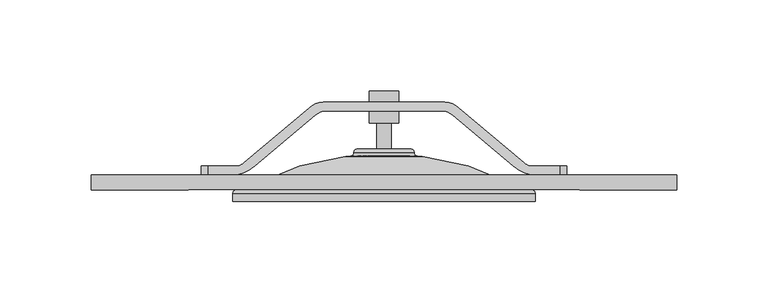
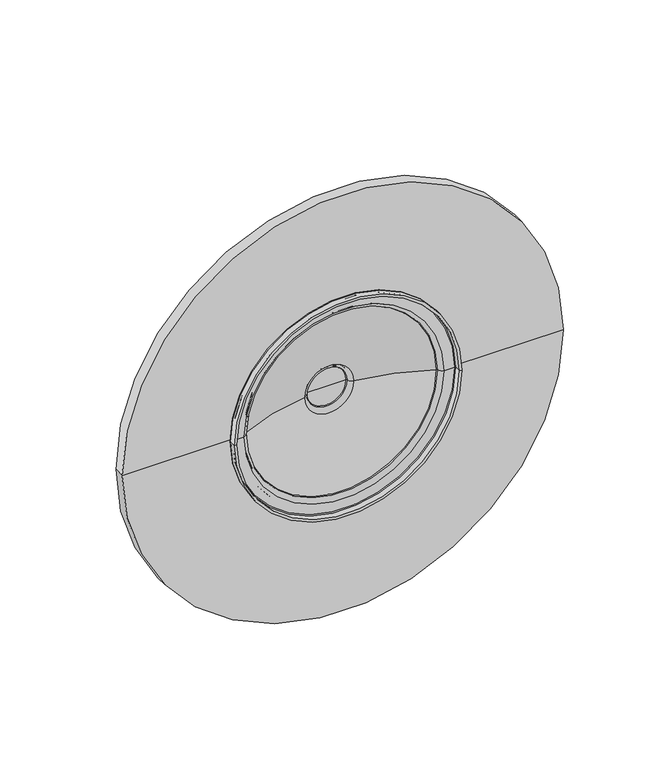
"""IFC4 building model written with IfcOpenShell, lengths in millimetres: proxy geometry, BVNC 300 8Y. : BVNC 300 8Y."""

from ifc_helpers import new_model, si_unit, point, frame, origin, place, context, project, spatial, polyline, circle_curve, ellipse_curve, trimmed, source, transform, mapped, element, save
from ifc_brep_helpers import plane_surface, cylinder_surface, revolved_surface, advanced_brep


def mechanical_equipment_492a67d3(model_context):
    return source(origin(), model_context, "Body", "AdvancedBrep", [
        advanced_brep(
        [(44.3795006, 108.0, 2610.0), (54.2298211, 113.0, 2610.0), (87.44309, 140.8692417, 2610.0), (91.8102497, 143.0, 2610.0), (125.0, 143.0, 2610.0), (158.1897503, 143.0, 2610.0), (162.55691, 140.8692417, 2610.0), (195.7701789, 113.0, 2610.0), (205.6204994, 108.0, 2610.0), (221.2200072, 108.0, 2610.0), (221.2200072, 113.0, 2610.0), (205.6204994, 113.0, 2610.0), (201.5540671, 114.8851429, 2610.0), (165.874925, 144.8234979, 2610.0), (158.1897503, 148.0, 2610.0), (125.0, 148.0, 2610.0), (91.8102497, 148.0, 2610.0), (84.125075, 144.8234979, 2610.0), (48.4459329, 114.8851429, 2610.0), (44.3795006, 113.0, 2610.0), (28.7799928, 113.0, 2610.0), (28.7799928, 108.0, 2610.0), (44.3795006, 113.0, 2590.0), (48.4459329, 114.8851429, 2590.0), (84.125075, 144.8234979, 2590.0), (91.8102497, 148.0, 2590.0), (125.0, 148.0, 2590.0), (158.1897503, 148.0, 2590.0), (165.874925, 144.8234979, 2590.0), (201.5540671, 114.8851429, 2590.0), (205.6204994, 113.0, 2590.0), (221.2200072, 113.0, 2590.0), (221.2200072, 108.0, 2590.0), (205.6204994, 108.0, 2590.0), (195.7701789, 113.0, 2590.0), (162.55691, 140.8692417, 2590.0), (158.1897503, 143.0, 2590.0), (125.0, 143.0, 2590.0), (91.8102497, 143.0, 2590.0), (87.44309, 140.8692417, 2590.0), (54.2298211, 113.0, 2590.0), (44.3795006, 108.0, 2590.0), (28.7799928, 108.0, 2590.0), (28.7799928, 113.0, 2590.0), (25.0, 108.0, 2606.2200072), (25.0, 108.0, 2593.7799928), (225.0, 108.0, 2593.7799928), (225.0, 108.0, 2606.2200072), (225.0, 113.0, 2593.7799928), (225.0, 113.0, 2606.2200072), (25.0, 113.0, 2593.7799928), (25.0, 113.0, 2606.2200072)],
        [
            (0, 1, circle_curve(frame((38.5511411, 131.6851233, 2610.0), z_axis=(0.0, 0.0, 1.0), x_axis=(1.0, 0.0, 0.0)), 24.3916961)),
            (1, 2),
            (2, 3, circle_curve(frame((93.9022065, 133.1715663, 2610.0), z_axis=(0.0, 0.0, -1.0), x_axis=(1.0, 0.0, 0.0)), 10.0486015)),
            (3, 4),
            (4, 5),
            (5, 6, circle_curve(frame((156.0977935, 133.1715663, 2610.0), z_axis=(0.0, 0.0, -1.0), x_axis=(-1.0, 0.0, 0.0)), 10.0486015)),
            (6, 7),
            (7, 8, circle_curve(frame((211.4488589, 131.6851233, 2610.0), z_axis=(0.0, 0.0, 1.0), x_axis=(-1.0, 0.0, 0.0)), 24.3916961)),
            (8, 9),
            (9, 10),
            (10, 11),
            (11, 12, circle_curve(frame((205.6204994, 118.3284116, 2610.0), z_axis=(0.0, 0.0, -1.0), x_axis=(-1.0, 0.0, 0.0)), 5.3284116)),
            (12, 13),
            (13, 14, circle_curve(frame((158.1897503, 137.115059, 2610.0), z_axis=(0.0, 0.0, 1.0), x_axis=(-1.0, 0.0, 0.0)), 10.884941)),
            (14, 15),
            (15, 16),
            (16, 17, circle_curve(frame((91.8102497, 137.115059, 2610.0), z_axis=(0.0, 0.0, 1.0), x_axis=(1.0, 0.0, 0.0)), 10.884941)),
            (17, 18),
            (18, 19, circle_curve(frame((44.3795006, 118.3284116, 2610.0), z_axis=(0.0, 0.0, -1.0), x_axis=(1.0, 0.0, 0.0)), 5.3284116)),
            (19, 20),
            (20, 21),
            (21, 0),
            (22, 23, circle_curve(frame((44.3795006, 118.3284116, 2590.0), z_axis=(0.0, 0.0, 1.0), x_axis=(1.0, 0.0, 0.0)), 5.3284116)),
            (23, 24),
            (24, 25, circle_curve(frame((91.8102497, 137.115059, 2590.0), z_axis=(0.0, 0.0, -1.0), x_axis=(1.0, 0.0, 0.0)), 10.884941)),
            (25, 26),
            (26, 27),
            (27, 28, circle_curve(frame((158.1897503, 137.115059, 2590.0), z_axis=(0.0, 0.0, -1.0), x_axis=(-1.0, 0.0, 0.0)), 10.884941)),
            (28, 29),
            (29, 30, circle_curve(frame((205.6204994, 118.3284116, 2590.0), z_axis=(0.0, 0.0, 1.0), x_axis=(-1.0, 0.0, 0.0)), 5.3284116)),
            (30, 31),
            (31, 32),
            (32, 33),
            (33, 34, circle_curve(frame((211.4488589, 131.6851233, 2590.0), z_axis=(0.0, 0.0, -1.0), x_axis=(-1.0, 0.0, 0.0)), 24.3916961)),
            (34, 35),
            (35, 36, circle_curve(frame((156.0977935, 133.1715663, 2590.0), z_axis=(0.0, 0.0, 1.0), x_axis=(-1.0, 0.0, 0.0)), 10.0486015)),
            (36, 37),
            (37, 38),
            (38, 39, circle_curve(frame((93.9022065, 133.1715663, 2590.0), z_axis=(0.0, 0.0, 1.0), x_axis=(1.0, 0.0, 0.0)), 10.0486015)),
            (39, 40),
            (40, 41, circle_curve(frame((38.5511411, 131.6851233, 2590.0), z_axis=(0.0, 0.0, -1.0), x_axis=(1.0, 0.0, 0.0)), 24.3916961)),
            (41, 42),
            (42, 43),
            (43, 22),
            (41, 0),
            (21, 44, circle_curve(frame((28.7799928, 108.0, 2606.2200072), z_axis=(0.0, -1.0, 0.0), x_axis=(1.0, 0.0, 0.0)), 3.7799928)),
            (44, 45),
            (45, 42, circle_curve(frame((28.7799928, 108.0, 2593.7799928), z_axis=(0.0, -1.0, 0.0), x_axis=(1.0, 0.0, 0.0)), 3.7799928)),
            (40, 1),
            (39, 2),
            (38, 3),
            (37, 4),
            (36, 5),
            (35, 6),
            (34, 7),
            (33, 8),
            (32, 46, circle_curve(frame((221.2200072, 108.0, 2593.7799928), z_axis=(0.0, -1.0, 0.0), x_axis=(-1.0, 0.0, 0.0)), 3.7799928)),
            (46, 47),
            (47, 9, circle_curve(frame((221.2200072, 108.0, 2606.2200072), z_axis=(0.0, -1.0, 0.0), x_axis=(-1.0, 0.0, 0.0)), 3.7799928)),
            (46, 48),
            (48, 49),
            (49, 47),
            (30, 11),
            (10, 49, circle_curve(frame((221.2200072, 113.0, 2606.2200072), z_axis=(0.0, 1.0, 0.0), x_axis=(-1.0, 0.0, 0.0)), 3.7799928)),
            (48, 31, circle_curve(frame((221.2200072, 113.0, 2593.7799928), z_axis=(0.0, 1.0, 0.0), x_axis=(-1.0, 0.0, 0.0)), 3.7799928)),
            (29, 12),
            (28, 13),
            (27, 14),
            (26, 15),
            (25, 16),
            (24, 17),
            (23, 18),
            (22, 19),
            (43, 50, circle_curve(frame((28.7799928, 113.0, 2593.7799928), z_axis=(0.0, 1.0, 0.0), x_axis=(1.0, 0.0, 0.0)), 3.7799928)),
            (50, 51),
            (51, 20, circle_curve(frame((28.7799928, 113.0, 2606.2200072), z_axis=(0.0, 1.0, 0.0), x_axis=(1.0, 0.0, 0.0)), 3.7799928)),
            (44, 51),
            (50, 45),
        ],
        [
            plane_surface(frame((25.0, 108.0, 2610.0), z_axis=(0.0, 0.0, 1.0), x_axis=(1.0, 0.0, 0.0))),
            plane_surface(frame((25.0, 108.0, 2590.0), z_axis=(0.0, 0.0, -1.0), x_axis=(-1.0, 0.0, 0.0))),
            plane_surface(frame((25.0, 108.0, 2610.0), z_axis=(0.0, -1.0, 0.0), x_axis=(0.0, 0.0, -1.0))),
            cylinder_surface(frame((38.5511411, 131.6851233, 2590.0), z_axis=(0.0, 0.0, 1.0), x_axis=(1.0, 0.0, 0.0)), 24.3916961),
            plane_surface(frame((54.2298211, 113.0, 2610.0), z_axis=(0.6427876096865391, -0.7660444431189783, 0.0), x_axis=(0.0, 0.0, -1.0))),
            revolved_surface(polyline([(103.95080800000001, 133.1715663, 2590.0), (103.95080800000001, 133.1715663, 2610.0)]), (93.9022065, 133.1715663, 2590.0), (0.0, 0.0, -1.0)),
            plane_surface(frame((91.8102497, 143.0, 2610.0), z_axis=(0.0, -1.0, 0.0), x_axis=(0.0, 0.0, -1.0))),
            plane_surface(frame((125.0, 143.0, 2610.0), z_axis=(0.0, -1.0, 0.0), x_axis=(0.0, 0.0, -1.0))),
            revolved_surface(polyline([(146.049192, 133.1715663, 2590.0), (146.049192, 133.1715663, 2610.0)]), (156.0977935, 133.1715663, 2590.0), (0.0, 0.0, -1.0)),
            plane_surface(frame((162.55691, 140.8692417, 2610.0), z_axis=(-0.6427876096865387, -0.7660444431189786, 0.0), x_axis=(0.0, 0.0, -1.0))),
            cylinder_surface(frame((211.4488589, 131.6851233, 2590.0), z_axis=(0.0, 0.0, 1.0), x_axis=(-1.0, 0.0, 0.0)), 24.3916961),
            plane_surface(frame((205.6204994, 108.0, 2610.0), z_axis=(0.0, -1.0, 0.0), x_axis=(0.0, 0.0, -1.0))),
            plane_surface(frame((225.0, 108.0, 2610.0), z_axis=(1.0, 0.0, 0.0), x_axis=(0.0, 0.0, -1.0))),
            plane_surface(frame((225.0, 113.0, 2610.0), z_axis=(0.0, 1.0, 0.0), x_axis=(0.0, 0.0, -1.0))),
            revolved_surface(polyline([(200.2920878, 118.3284116, 2590.0), (200.2920878, 118.3284116, 2610.0)]), (205.6204994, 118.3284116, 2590.0), (0.0, 0.0, -1.0)),
            plane_surface(frame((201.5540671, 114.8851429, 2610.0), z_axis=(0.6427876096865414, 0.7660444431189763, 0.0), x_axis=(0.0, 0.0, -1.0))),
            cylinder_surface(frame((158.1897503, 137.115059, 2590.0), z_axis=(0.0, 0.0, 1.0), x_axis=(-1.0, 0.0, 0.0)), 10.884941),
            plane_surface(frame((158.1897503, 148.0, 2610.0), z_axis=(0.0, 1.0, 0.0), x_axis=(0.0, 0.0, -1.0))),
            plane_surface(frame((125.0, 148.0, 2610.0), z_axis=(0.0, 1.0, 0.0), x_axis=(0.0, 0.0, -1.0))),
            cylinder_surface(frame((91.8102497, 137.115059, 2590.0), z_axis=(0.0, 0.0, 1.0), x_axis=(1.0, 0.0, 0.0)), 10.884941),
            plane_surface(frame((84.125075, 144.8234979, 2610.0), z_axis=(-0.6427876096865359, 0.766044443118981, 0.0), x_axis=(0.0, 0.0, -1.0))),
            revolved_surface(polyline([(49.7079122, 118.3284116, 2590.0), (49.7079122, 118.3284116, 2610.0)]), (44.3795006, 118.3284116, 2590.0), (0.0, 0.0, -1.0)),
            plane_surface(frame((44.3795006, 113.0, 2610.0), z_axis=(0.0, 1.0, 0.0), x_axis=(0.0, 0.0, -1.0))),
            plane_surface(frame((25.0, 113.0, 2610.0), z_axis=(-1.0, 0.0, 0.0), x_axis=(0.0, 0.0, -1.0))),
            cylinder_surface(frame((28.7799928, 108.0, 2593.7799928), z_axis=(0.0, -1.0, 0.0), x_axis=(1.0, 0.0, 0.0)), 3.7799928),
            cylinder_surface(frame((28.7799928, 93.5, 2606.2200072), z_axis=(0.0, -1.0, 0.0), x_axis=(1.0, 0.0, 0.0)), 3.7799928),
            cylinder_surface(frame((221.2200072, 93.5, 2593.7799928), z_axis=(0.0, -1.0, 0.0), x_axis=(-1.0, 0.0, 0.0)), 3.7799928),
            cylinder_surface(frame((221.2200072, 93.5, 2606.2200072), z_axis=(0.0, -1.0, 0.0), x_axis=(-1.0, 0.0, 0.0)), 3.7799928),
        ],
        [
            (0, [[1, 2, 3, 4, 5, 6, 7, 8, 9, 10, 11, 12, 13, 14, 15, 16, 17, 18, 19, 20, 21, 22]]),
            (1, [[23, 24, 25, 26, 27, 28, 29, 30, 31, 32, 33, 34, 35, 36, 37, 38, 39, 40, 41, 42, 43, 44]]),
            (2, [[45, -22, 46, 47, 48, -42]]),
            (3, [[-1, -45, -41, 49]]),
            (4, [[-2, -49, -40, 50]]),
            (5, [[-3, -50, -39, 51]]),
            (6, [[-4, -51, -38, 52]]),
            (7, [[-5, -52, -37, 53]]),
            (8, [[-6, -53, -36, 54]]),
            (9, [[-7, -54, -35, 55]]),
            (10, [[-8, -55, -34, 56]]),
            (11, [[-56, -33, 57, 58, 59, -9]]),
            (12, [[-58, 60, 61, 62]]),
            (13, [[63, -11, 64, -61, 65, -31]]),
            (14, [[-12, -63, -30, 66]]),
            (15, [[-13, -66, -29, 67]]),
            (16, [[-14, -67, -28, 68]]),
            (17, [[-15, -68, -27, 69]]),
            (18, [[-16, -69, -26, 70]]),
            (19, [[-17, -70, -25, 71]]),
            (20, [[-18, -71, -24, 72]]),
            (21, [[-19, -72, -23, 73]]),
            (22, [[-73, -44, 74, 75, 76, -20]]),
            (23, [[-47, 77, -75, 78]]),
            (24, [[-43, -48, -78, -74]]),
            (25, [[-21, -76, -77, -46]]),
            (26, [[-32, -65, -60, -57]]),
            (27, [[-10, -59, -62, -64]]),
        ],
    ),
        advanced_brep(
        [(207.7271571, 93.5, 2600.0), (42.2728429, 93.5, 2600.0), (42.2728429, 97.7728429, 2600.0), (207.7271571, 97.7728429, 2600.0), (205.9367462, 93.5, 2600.0), (44.0632538, 93.5, 2600.0), (205.9367462, 97.9071057, 2600.0), (44.0632538, 97.9071057, 2600.0), (205.3438519, 98.5, 2600.0), (44.6561481, 98.5, 2600.0), (197.7785514, 98.5, 2600.0), (52.2214486, 98.5, 2600.0), (194.5390342, 101.1233093, 2600.0), (55.4609658, 101.1233093, 2600.0), (194.110594, 101.9290881, 2600.0), (55.889406, 101.9290881, 2600.0), (143.1174907, 117.056758, 2600.0), (106.8825093, 117.056758, 2600.0), (139.9690463, 120.2052024, 2600.0), (110.0309537, 120.2052024, 2600.0), (139.3942487, 120.78, 2600.0), (110.6057513, 120.78, 2600.0), (125.0, 120.78, 2600.0), (139.6388233, 122.2731901, 2600.0), (110.3611767, 122.2731901, 2600.0), (120.9566338, 122.2731901, 2600.0), (129.0433662, 122.2731901, 2600.0), (141.5029828, 120.4090307, 2600.0), (108.4970172, 120.4090307, 2600.0), (143.1991524, 118.522856, 2600.0), (106.8008476, 118.522856, 2600.0), (145.9642188, 118.2410596, 2600.0), (104.0357812, 118.2410596, 2600.0), (194.877574, 103.206216, 2600.0), (55.122426, 103.206216, 2600.0), (196.1038029, 101.6367146, 2600.0), (53.8961971, 101.6367146, 2600.0), (198.0543634, 100.0, 2600.0), (51.9456366, 100.0, 2600.0), (200.0, 100.0, 2600.0), (50.0, 100.0, 2600.0), (200.0, 108.0, 2600.0), (50.0, 108.0, 2600.0), (285.0, 108.0, 2600.0), (-35.0, 108.0, 2600.0), (285.0, 100.0, 2600.0), (-35.0, 100.0, 2600.0), (205.5, 100.0, 2600.0), (44.5, 100.0, 2600.0), (133.0867323, 136.6576943, 2600.0), (116.9132677, 136.6576943, 2600.0), (116.9132677, 153.9, 2600.0), (133.0867323, 153.9, 2600.0), (129.0433662, 136.6576943, 2600.0), (120.9566338, 136.6576943, 2600.0), (125.0, 153.9, 2600.0)],
        [
            (0, 1, circle_curve(frame((125.0, 93.5, 2600.0), z_axis=(0.0, 1.0, 0.0), x_axis=(-1.0, 0.0, 0.0)), 82.7271571)),
            (1, 2),
            (2, 3, circle_curve(frame((125.0, 97.7728429, 2600.0), z_axis=(0.0, -1.0, 0.0), x_axis=(-1.0, 0.0, 0.0)), 82.7271571)),
            (3, 0),
            (1, 0, circle_curve(frame((125.0, 93.5, 2600.0), z_axis=(0.0, 1.0, 0.0), x_axis=(-1.0, 0.0, 0.0)), 82.7271571)),
            (3, 2, circle_curve(frame((125.0, 97.7728429, 2600.0), z_axis=(0.0, -1.0, 0.0), x_axis=(-1.0, 0.0, 0.0)), 82.7271571)),
            (0, 4),
            (4, 5, circle_curve(frame((125.0, 93.5, 2600.0), z_axis=(0.0, 1.0, 0.0), x_axis=(-1.0, 0.0, 0.0)), 80.9367462)),
            (5, 1),
            (5, 4, circle_curve(frame((125.0, 93.5, 2600.0), z_axis=(0.0, 1.0, 0.0), x_axis=(-1.0, 0.0, 0.0)), 80.9367462)),
            (4, 6),
            (6, 7, circle_curve(frame((125.0, 97.9071057, 2600.0), z_axis=(0.0, 1.0, 0.0), x_axis=(-1.0, 0.0, 0.0)), 80.9367462)),
            (7, 5),
            (7, 6, circle_curve(frame((125.0, 97.9071057, 2600.0), z_axis=(0.0, 1.0, 0.0), x_axis=(-1.0, 0.0, 0.0)), 80.9367462)),
            (6, 8, circle_curve(frame((205.3438519, 97.9071057, 2600.0), z_axis=(0.0, 0.0, 1.0), x_axis=(-1.0, 0.0, 0.0)), 0.5928943)),
            (8, 9, circle_curve(frame((125.0, 98.5, 2600.0), z_axis=(0.0, 1.0, 0.0), x_axis=(-1.0, 0.0, 0.0)), 80.3438519)),
            (9, 7, circle_curve(frame((44.6561481, 97.9071057, 2600.0), z_axis=(0.0, 0.0, 1.0), x_axis=(1.0, 0.0, 0.0)), 0.5928943)),
            (9, 8, circle_curve(frame((125.0, 98.5, 2600.0), z_axis=(0.0, 1.0, 0.0), x_axis=(-1.0, 0.0, 0.0)), 80.3438519)),
            (8, 10),
            (10, 11, circle_curve(frame((125.0, 98.5, 2600.0), z_axis=(0.0, 1.0, 0.0), x_axis=(-1.0, 0.0, 0.0)), 72.7785514)),
            (11, 9),
            (11, 10, circle_curve(frame((125.0, 98.5, 2600.0), z_axis=(0.0, 1.0, 0.0), x_axis=(-1.0, 0.0, 0.0)), 72.7785514)),
            (10, 12, circle_curve(frame((197.9467336, 102.0195777, 2600.0), z_axis=(0.0, 0.0, -1.0), x_axis=(-1.0, 0.0, 0.0)), 3.5235937)),
            (12, 13, circle_curve(frame((125.0, 101.1233093, 2600.0), z_axis=(0.0, 1.0, 0.0), x_axis=(-1.0, 0.0, 0.0)), 69.5390342)),
            (13, 11, circle_curve(frame((52.0532664, 102.0195777, 2600.0), z_axis=(0.0, 0.0, -1.0), x_axis=(1.0, 0.0, 0.0)), 3.5235937)),
            (13, 12, circle_curve(frame((125.0, 101.1233093, 2600.0), z_axis=(0.0, 1.0, 0.0), x_axis=(-1.0, 0.0, 0.0)), 69.5390342)),
            (12, 14, circle_curve(frame((193.7458269, 101.2183458, 2600.0), z_axis=(0.0, 0.0, 1.0), x_axis=(-1.0, 0.0, 0.0)), 0.7988803)),
            (14, 15, circle_curve(frame((125.0, 101.9290881, 2600.0), z_axis=(0.0, 1.0, 0.0), x_axis=(-1.0, 0.0, 0.0)), 69.110594)),
            (15, 13, circle_curve(frame((56.2541731, 101.2183458, 2600.0), z_axis=(0.0, 0.0, 1.0), x_axis=(1.0, 0.0, 0.0)), 0.7988803)),
            (15, 14, circle_curve(frame((125.0, 101.9290881, 2600.0), z_axis=(0.0, 1.0, 0.0), x_axis=(-1.0, 0.0, 0.0)), 69.110594)),
            (14, 16, circle_curve(frame((128.3688639, -26.1675298, 2600.0), z_axis=(0.0, 0.0, 1.0), x_axis=(-1.0, 0.0, 0.0)), 143.9816606)),
            (16, 17, circle_curve(frame((125.0, 117.056758, 2600.0), z_axis=(0.0, 1.0, 0.0), x_axis=(-1.0, 0.0, 0.0)), 18.1174907)),
            (17, 15, circle_curve(frame((121.6311361, -26.1675298, 2600.0), z_axis=(0.0, 0.0, 1.0), x_axis=(1.0, 0.0, 0.0)), 143.9816606)),
            (17, 16, circle_curve(frame((125.0, 117.056758, 2600.0), z_axis=(0.0, 1.0, 0.0), x_axis=(-1.0, 0.0, 0.0)), 18.1174907)),
            (16, 18, circle_curve(frame((143.1174907, 120.2052024, 2600.0), z_axis=(0.0, 0.0, -1.0), x_axis=(-1.0, 0.0, 0.0)), 3.1484444)),
            (18, 19, circle_curve(frame((125.0, 120.2052024, 2600.0), z_axis=(0.0, 1.0, 0.0), x_axis=(-1.0, 0.0, 0.0)), 14.9690463)),
            (19, 17, circle_curve(frame((106.8825093, 120.2052024, 2600.0), z_axis=(0.0, 0.0, -1.0), x_axis=(1.0, 0.0, 0.0)), 3.1484444)),
            (19, 18, circle_curve(frame((125.0, 120.2052024, 2600.0), z_axis=(0.0, 1.0, 0.0), x_axis=(-1.0, 0.0, 0.0)), 14.9690463)),
            (18, 20, circle_curve(frame((139.3942487, 120.2052024, 2600.0), z_axis=(0.0, 0.0, 1.0), x_axis=(-1.0, 0.0, 0.0)), 0.5747976)),
            (20, 21, circle_curve(frame((125.0, 120.78, 2600.0), z_axis=(0.0, 1.0, 0.0), x_axis=(-1.0, 0.0, 0.0)), 14.3942487)),
            (21, 19, circle_curve(frame((110.6057513, 120.2052024, 2600.0), z_axis=(0.0, 0.0, 1.0), x_axis=(1.0, 0.0, 0.0)), 0.5747976)),
            (21, 20, circle_curve(frame((125.0, 120.78, 2600.0), z_axis=(0.0, 1.0, 0.0), x_axis=(-1.0, 0.0, 0.0)), 14.3942487)),
            (20, 22),
            (22, 21),
            (23, 24, circle_curve(frame((125.0, 122.2731901, 2600.0), z_axis=(0.0, 1.0, 0.0), x_axis=(-1.0, 0.0, 0.0)), 14.6388233)),
            (24, 25),
            (25, 26, circle_curve(frame((125.0, 122.2731901, 2600.0), z_axis=(0.0, -1.0, 0.0), x_axis=(-1.0, 0.0, 0.0)), 4.0433662)),
            (26, 23),
            (24, 23, circle_curve(frame((125.0, 122.2731901, 2600.0), z_axis=(0.0, 1.0, 0.0), x_axis=(-1.0, 0.0, 0.0)), 14.6388233)),
            (26, 25, circle_curve(frame((125.0, 122.2731901, 2600.0), z_axis=(0.0, -1.0, 0.0), x_axis=(-1.0, 0.0, 0.0)), 4.0433662)),
            (23, 27, circle_curve(frame((139.6388233, 120.4090307, 2600.0), z_axis=(0.0, 0.0, -1.0), x_axis=(-1.0, 0.0, 0.0)), 1.8641595)),
            (27, 28, circle_curve(frame((125.0, 120.4090307, 2600.0), z_axis=(0.0, 1.0, 0.0), x_axis=(-1.0, 0.0, 0.0)), 16.5029828)),
            (28, 24, circle_curve(frame((110.3611767, 120.4090307, 2600.0), z_axis=(0.0, 0.0, -1.0), x_axis=(1.0, 0.0, 0.0)), 1.8641595)),
            (28, 27, circle_curve(frame((125.0, 120.4090307, 2600.0), z_axis=(0.0, 1.0, 0.0), x_axis=(-1.0, 0.0, 0.0)), 16.5029828)),
            (27, 29, circle_curve(frame((143.3997997, 120.4090307, 2600.0), z_axis=(0.0, 0.0, 1.0), x_axis=(-1.0, 0.0, 0.0)), 1.8968169)),
            (29, 30, circle_curve(frame((125.0, 118.522856, 2600.0), z_axis=(0.0, 1.0, 0.0), x_axis=(-1.0, 0.0, 0.0)), 18.1991524)),
            (30, 28, circle_curve(frame((106.6002003, 120.4090307, 2600.0), z_axis=(0.0, 0.0, 1.0), x_axis=(1.0, 0.0, 0.0)), 1.8968169)),
            (30, 29, circle_curve(frame((125.0, 118.522856, 2600.0), z_axis=(0.0, 1.0, 0.0), x_axis=(-1.0, 0.0, 0.0)), 18.1991524)),
            (29, 31, circle_curve(frame((176.4809645, 431.386753, 2600.0), z_axis=(0.0, 0.0, 1.0), x_axis=(-1.0, 0.0, 0.0)), 314.6291421)),
            (31, 32, circle_curve(frame((125.0, 118.2410596, 2600.0), z_axis=(0.0, 1.0, 0.0), x_axis=(-1.0, 0.0, 0.0)), 20.9642188)),
            (32, 30, circle_curve(frame((73.5190355, 431.386753, 2600.0), z_axis=(0.0, 0.0, 1.0), x_axis=(1.0, 0.0, 0.0)), 314.6291421)),
            (32, 31, circle_curve(frame((125.0, 118.2410596, 2600.0), z_axis=(0.0, 1.0, 0.0), x_axis=(-1.0, 0.0, 0.0)), 20.9642188)),
            (31, 33, circle_curve(frame((131.9555378, -14.4169888, 2600.0), z_axis=(0.0, 0.0, -1.0), x_axis=(-1.0, 0.0, 0.0)), 133.3956557)),
            (33, 34, circle_curve(frame((125.0, 103.206216, 2600.0), z_axis=(0.0, 1.0, 0.0), x_axis=(-1.0, 0.0, 0.0)), 69.877574)),
            (34, 32, circle_curve(frame((118.0444622, -14.4169888, 2600.0), z_axis=(0.0, 0.0, -1.0), x_axis=(1.0, 0.0, 0.0)), 133.3956557)),
            (34, 33, circle_curve(frame((125.0, 103.206216, 2600.0), z_axis=(0.0, 1.0, 0.0), x_axis=(-1.0, 0.0, 0.0)), 69.877574)),
            (33, 35, circle_curve(frame((194.0147871, 101.2683648, 2600.0), z_axis=(0.0, 0.0, -1.0), x_axis=(-1.0, 0.0, 0.0)), 2.1212422)),
            (35, 36, circle_curve(frame((125.0, 101.6367146, 2600.0), z_axis=(0.0, 1.0, 0.0), x_axis=(-1.0, 0.0, 0.0)), 71.1038029)),
            (36, 34, circle_curve(frame((55.9852129, 101.2683648, 2600.0), z_axis=(0.0, 0.0, -1.0), x_axis=(1.0, 0.0, 0.0)), 2.1212422)),
            (36, 35, circle_curve(frame((125.0, 101.6367146, 2600.0), z_axis=(0.0, 1.0, 0.0), x_axis=(-1.0, 0.0, 0.0)), 71.1038029)),
            (35, 37, circle_curve(frame((198.0543634, 101.9806511, 2600.0), z_axis=(0.0, 0.0, 1.0), x_axis=(-1.0, 0.0, 0.0)), 1.9806511)),
            (37, 38, circle_curve(frame((125.0, 100.0, 2600.0), z_axis=(0.0, 1.0, 0.0), x_axis=(-1.0, 0.0, 0.0)), 73.0543634)),
            (38, 36, circle_curve(frame((51.9456366, 101.9806511, 2600.0), z_axis=(0.0, 0.0, 1.0), x_axis=(1.0, 0.0, 0.0)), 1.9806511)),
            (38, 37, circle_curve(frame((125.0, 100.0, 2600.0), z_axis=(0.0, 1.0, 0.0), x_axis=(-1.0, 0.0, 0.0)), 73.0543634)),
            (37, 39),
            (39, 40, circle_curve(frame((125.0, 100.0, 2600.0), z_axis=(0.0, 1.0, 0.0), x_axis=(-1.0, 0.0, 0.0)), 75.0)),
            (40, 38),
            (40, 39, circle_curve(frame((125.0, 100.0, 2600.0), z_axis=(0.0, 1.0, 0.0), x_axis=(-1.0, 0.0, 0.0)), 75.0)),
            (39, 41),
            (41, 42, circle_curve(frame((125.0, 108.0, 2600.0), z_axis=(0.0, 1.0, 0.0), x_axis=(-1.0, 0.0, 0.0)), 75.0)),
            (42, 40),
            (42, 41, circle_curve(frame((125.0, 108.0, 2600.0), z_axis=(0.0, 1.0, 0.0), x_axis=(-1.0, 0.0, 0.0)), 75.0)),
            (41, 43),
            (43, 44, circle_curve(frame((125.0, 108.0, 2600.0), z_axis=(0.0, 1.0, 0.0), x_axis=(-1.0, 0.0, 0.0)), 160.0)),
            (44, 42),
            (44, 43, circle_curve(frame((125.0, 108.0, 2600.0), z_axis=(0.0, 1.0, 0.0), x_axis=(-1.0, 0.0, 0.0)), 160.0)),
            (43, 45),
            (45, 46, circle_curve(frame((125.0, 100.0, 2600.0), z_axis=(0.0, 1.0, 0.0), x_axis=(-1.0, 0.0, 0.0)), 160.0)),
            (46, 44),
            (46, 45, circle_curve(frame((125.0, 100.0, 2600.0), z_axis=(0.0, 1.0, 0.0), x_axis=(-1.0, 0.0, 0.0)), 160.0)),
            (45, 47),
            (47, 48, circle_curve(frame((125.0, 100.0, 2600.0), z_axis=(0.0, 1.0, 0.0), x_axis=(-1.0, 0.0, 0.0)), 80.5)),
            (48, 46),
            (48, 47, circle_curve(frame((125.0, 100.0, 2600.0), z_axis=(0.0, 1.0, 0.0), x_axis=(-1.0, 0.0, 0.0)), 80.5)),
            (2, 48, circle_curve(frame((44.5, 97.7728429, 2600.0), z_axis=(0.0, 0.0, -1.0), x_axis=(1.0, 0.0, 0.0)), 2.2271571)),
            (47, 3, circle_curve(frame((205.5, 97.7728429, 2600.0), z_axis=(0.0, 0.0, -1.0), x_axis=(-1.0, 0.0, 0.0)), 2.2271571)),
            (49, 50, circle_curve(frame((125.0, 136.6576943, 2600.0), z_axis=(0.0, 1.0, 0.0), x_axis=(-1.0, 0.0, 0.0)), 8.0867323)),
            (50, 51),
            (51, 52, circle_curve(frame((125.0, 153.9, 2600.0), z_axis=(0.0, -1.0, 0.0), x_axis=(-1.0, 0.0, 0.0)), 8.0867323)),
            (52, 49),
            (50, 49, circle_curve(frame((125.0, 136.6576943, 2600.0), z_axis=(0.0, 1.0, 0.0), x_axis=(-1.0, 0.0, 0.0)), 8.0867323)),
            (52, 51, circle_curve(frame((125.0, 153.9, 2600.0), z_axis=(0.0, -1.0, 0.0), x_axis=(-1.0, 0.0, 0.0)), 8.0867323)),
            (49, 53),
            (53, 54, circle_curve(frame((125.0, 136.6576943, 2600.0), z_axis=(0.0, 1.0, 0.0), x_axis=(-1.0, 0.0, 0.0)), 4.0433662)),
            (54, 50),
            (54, 53, circle_curve(frame((125.0, 136.6576943, 2600.0), z_axis=(0.0, 1.0, 0.0), x_axis=(-1.0, 0.0, 0.0)), 4.0433662)),
            (51, 55),
            (55, 52),
            (25, 54),
            (53, 26),
        ],
        [
            cylinder_surface(frame((125.0, 193.5, 2600.0), z_axis=(0.0, -1.0, 0.0), x_axis=(-1.0, 0.0, 0.0)), 82.7271571),
            plane_surface(frame((125.0, 93.5, 2600.0), z_axis=(0.0, -1.0, 0.0), x_axis=(-1.0, 0.0, 0.0))),
            revolved_surface(polyline([(44.0632538, 93.5, 2600.0), (44.0632538, 97.9071057, 2600.0)]), (125.0, 193.5, 2600.0), (0.0, -1.0, 0.0)),
            revolved_surface(trimmed(ellipse_curve(frame((44.6561481, 97.9071057, 2600.0), z_axis=(0.0, 0.0, -1.0), x_axis=(1.0, 0.0, 0.0)), 0.5928943, 0.5928943), [point((44.0632538, 97.9071057, 2600.0))], [point((44.6561481, 98.5, 2600.0))], True, "CARTESIAN"), (125.0, 193.5, 2600.0), (0.0, -1.0, 0.0)),
            plane_surface(frame((125.0, 98.5, 2600.0), z_axis=(0.0, -1.0, 0.0), x_axis=(-1.0, 0.0, 0.0))),
            revolved_surface(trimmed(ellipse_curve(frame((52.0532664, 102.0195777, 2600.0), z_axis=(0.0, 0.0, 1.0), x_axis=(1.0, 0.0, 0.0)), 3.5235937, 3.5235937), [point((52.2214486, 98.5, 2600.0))], [point((55.4609658, 101.1233093, 2600.0))], True, "CARTESIAN"), (125.0, 193.5, 2600.0), (0.0, -1.0, 0.0)),
            revolved_surface(trimmed(ellipse_curve(frame((56.2541731, 101.2183458, 2600.0), z_axis=(0.0, 0.0, -1.0), x_axis=(1.0, 0.0, 0.0)), 0.7988803, 0.7988803), [point((55.4609658, 101.1233093, 2600.0))], [point((55.889406, 101.9290881, 2600.0))], True, "CARTESIAN"), (125.0, 193.5, 2600.0), (0.0, -1.0, 0.0)),
            revolved_surface(trimmed(ellipse_curve(frame((121.6311361, -26.1675298, 2600.0), z_axis=(0.0, 0.0, -1.0), x_axis=(1.0, 0.0, 0.0)), 143.9816606, 143.9816606), [point((55.889406, 101.9290881, 2600.0))], [point((106.8825093, 117.056758, 2600.0))], True, "CARTESIAN"), (125.0, 193.5, 2600.0), (0.0, -1.0, 0.0)),
            revolved_surface(trimmed(ellipse_curve(frame((106.8825093, 120.2052024, 2600.0), z_axis=(0.0, 0.0, 1.0), x_axis=(1.0, 0.0, 0.0)), 3.1484444, 3.1484444), [point((106.8825093, 117.056758, 2600.0))], [point((110.0309537, 120.2052024, 2600.0))], True, "CARTESIAN"), (125.0, 193.5, 2600.0), (0.0, -1.0, 0.0)),
            revolved_surface(trimmed(ellipse_curve(frame((110.6057513, 120.2052024, 2600.0), z_axis=(0.0, 0.0, -1.0), x_axis=(1.0, 0.0, 0.0)), 0.5747976, 0.5747976), [point((110.0309537, 120.2052024, 2600.0))], [point((110.6057513, 120.78, 2600.0))], True, "CARTESIAN"), (125.0, 193.5, 2600.0), (0.0, -1.0, 0.0)),
            plane_surface(frame((125.0, 120.78, 2600.0), z_axis=(0.0, -1.0, 0.0), x_axis=(-1.0, 0.0, 0.0))),
            plane_surface(frame((125.0, 122.2731901, 2600.0), z_axis=(0.0, 1.0, 0.0), x_axis=(-1.0, 0.0, 0.0))),
            revolved_surface(trimmed(ellipse_curve(frame((110.3611767, 120.4090307, 2600.0), z_axis=(0.0, 0.0, 1.0), x_axis=(1.0, 0.0, 0.0)), 1.8641595, 1.8641595), [point((110.3611767, 122.2731901, 2600.0))], [point((108.4970172, 120.4090307, 2600.0))], True, "CARTESIAN"), (125.0, 193.5, 2600.0), (0.0, -1.0, 0.0)),
            revolved_surface(trimmed(ellipse_curve(frame((106.6002003, 120.4090307, 2600.0), z_axis=(0.0, 0.0, -1.0), x_axis=(1.0, 0.0, 0.0)), 1.8968169, 1.8968169), [point((108.4970172, 120.4090307, 2600.0))], [point((106.8008476, 118.522856, 2600.0))], True, "CARTESIAN"), (125.0, 193.5, 2600.0), (0.0, -1.0, 0.0)),
            revolved_surface(trimmed(ellipse_curve(frame((73.5190355, 431.386753, 2600.0), z_axis=(0.0, 0.0, -1.0), x_axis=(1.0, 0.0, 0.0)), 314.6291421, 314.6291421), [point((106.8008476, 118.522856, 2600.0))], [point((104.0357812, 118.2410596, 2600.0))], True, "CARTESIAN"), (125.0, 193.5, 2600.0), (0.0, -1.0, 0.0)),
            revolved_surface(trimmed(ellipse_curve(frame((118.0444622, -14.4169888, 2600.0), z_axis=(0.0, 0.0, 1.0), x_axis=(1.0, 0.0, 0.0)), 133.3956557, 133.3956557), [point((104.0357812, 118.2410596, 2600.0))], [point((55.122426, 103.206216, 2600.0))], True, "CARTESIAN"), (125.0, 193.5, 2600.0), (0.0, -1.0, 0.0)),
            revolved_surface(trimmed(ellipse_curve(frame((55.9852129, 101.2683648, 2600.0), z_axis=(0.0, 0.0, 1.0), x_axis=(1.0, 0.0, 0.0)), 2.1212422, 2.1212422), [point((55.122426, 103.206216, 2600.0))], [point((53.8961971, 101.6367146, 2600.0))], True, "CARTESIAN"), (125.0, 193.5, 2600.0), (0.0, -1.0, 0.0)),
            revolved_surface(trimmed(ellipse_curve(frame((51.9456366, 101.9806511, 2600.0), z_axis=(0.0, 0.0, -1.0), x_axis=(1.0, 0.0, 0.0)), 1.9806511, 1.9806511), [point((53.8961971, 101.6367146, 2600.0))], [point((51.9456366, 100.0, 2600.0))], True, "CARTESIAN"), (125.0, 193.5, 2600.0), (0.0, -1.0, 0.0)),
            plane_surface(frame((125.0, 100.0, 2600.0), z_axis=(0.0, 1.0, 0.0), x_axis=(-1.0, 0.0, 0.0))),
            revolved_surface(polyline([(50.0, 100.0, 2600.0), (50.0, 108.0, 2600.0)]), (125.0, 193.5, 2600.0), (0.0, -1.0, 0.0)),
            plane_surface(frame((125.0, 108.0, 2600.0), z_axis=(0.0, 1.0, 0.0), x_axis=(-1.0, 0.0, 0.0))),
            cylinder_surface(frame((125.0, 193.5, 2600.0), z_axis=(0.0, -1.0, 0.0), x_axis=(-1.0, 0.0, 0.0)), 160.0),
            plane_surface(frame((125.0, 100.0, 2600.0), z_axis=(0.0, -1.0, 0.0), x_axis=(-1.0, 0.0, 0.0))),
            revolved_surface(trimmed(ellipse_curve(frame((44.5, 97.7728429, 2600.0), z_axis=(0.0, 0.0, 1.0), x_axis=(1.0, 0.0, 0.0)), 2.2271571, 2.2271571), [point((44.5, 100.0, 2600.0))], [point((42.2728429, 97.7728429, 2600.0))], True, "CARTESIAN"), (125.0, 193.5, 2600.0), (0.0, -1.0, 0.0)),
            cylinder_surface(frame((125.0, 193.5, 2600.0), z_axis=(0.0, -1.0, 0.0), x_axis=(-1.0, 0.0, 0.0)), 8.0867323),
            plane_surface(frame((125.0, 136.6576943, 2600.0), z_axis=(0.0, -1.0, 0.0), x_axis=(-1.0, 0.0, 0.0))),
            plane_surface(frame((125.0, 153.9, 2600.0), z_axis=(0.0, 1.0, 0.0), x_axis=(-1.0, 0.0, 0.0))),
            cylinder_surface(frame((125.0, 193.5, 2600.0), z_axis=(0.0, -1.0, 0.0), x_axis=(-1.0, 0.0, 0.0)), 4.0433662),
        ],
        [
            (0, [[1, 2, 3, 4]]),
            (0, [[-2, 5, -4, 6]]),
            (1, [[-1, 7, 8, 9]]),
            (1, [[-5, -9, 10, -7]]),
            (2, [[-8, 11, 12, 13]]),
            (2, [[-10, -13, 14, -11]]),
            (3, [[-12, 15, 16, 17]]),
            (3, [[-14, -17, 18, -15]]),
            (4, [[-16, 19, 20, 21]]),
            (4, [[-18, -21, 22, -19]]),
            (5, [[-20, 23, 24, 25]]),
            (5, [[-22, -25, 26, -23]]),
            (6, [[-24, 27, 28, 29]]),
            (6, [[-26, -29, 30, -27]]),
            (7, [[-28, 31, 32, 33]]),
            (7, [[-30, -33, 34, -31]]),
            (8, [[-32, 35, 36, 37]]),
            (8, [[-34, -37, 38, -35]]),
            (9, [[-36, 39, 40, 41]]),
            (9, [[-38, -41, 42, -39]]),
            (10, [[-40, 43, 44]]),
            (10, [[-42, -44, -43]]),
            (11, [[45, 46, 47, 48]]),
            (11, [[-46, 49, -48, 50]]),
            (12, [[-45, 51, 52, 53]]),
            (12, [[-49, -53, 54, -51]]),
            (13, [[-52, 55, 56, 57]]),
            (13, [[-54, -57, 58, -55]]),
            (14, [[-56, 59, 60, 61]]),
            (14, [[-58, -61, 62, -59]]),
            (15, [[-60, 63, 64, 65]]),
            (15, [[-62, -65, 66, -63]]),
            (16, [[-64, 67, 68, 69]]),
            (16, [[-66, -69, 70, -67]]),
            (17, [[-68, 71, 72, 73]]),
            (17, [[-70, -73, 74, -71]]),
            (18, [[-72, 75, 76, 77]]),
            (18, [[-74, -77, 78, -75]]),
            (19, [[-76, 79, 80, 81]]),
            (19, [[-78, -81, 82, -79]]),
            (20, [[-80, 83, 84, 85]]),
            (20, [[-82, -85, 86, -83]]),
            (21, [[-84, 87, 88, 89]]),
            (21, [[-86, -89, 90, -87]]),
            (22, [[-88, 91, 92, 93]]),
            (22, [[-90, -93, 94, -91]]),
            (23, [[-3, 95, -92, 96]]),
            (23, [[-6, -96, -94, -95]]),
            (24, [[97, 98, 99, 100]]),
            (24, [[-98, 101, -100, 102]]),
            (25, [[-97, 103, 104, 105]]),
            (25, [[-101, -105, 106, -103]]),
            (26, [[-99, 107, 108]]),
            (26, [[-102, -108, -107]]),
            (27, [[-47, 109, -104, 110]]),
            (27, [[-50, -110, -106, -109]]),
        ],
    ),
    ])


if __name__ == "__main__":
    model = new_model("IFC4")
    model_context = context("Model", 3, world=origin())
    ifc_project = project(units=[si_unit("LENGTHUNIT", "METRE", prefix="MILLI")], contexts=[model_context])
    site = spatial("IfcSite", under=ifc_project)
    building = spatial("IfcBuilding", under=site)
    placement = place(None, origin())
    mechanical_equipment_shape = mechanical_equipment_492a67d3(model_context)
    element("IfcBuildingElementProxy", 1, Name="BVNC 300 8Y. : BVNC 300 8Y", ObjectType="BVNC 300 8Y. : BVNC 300 8Y", at=placement, inside=building, context=model_context, shape_type="MappedRepresentation", body=[
        mapped(mechanical_equipment_shape, transform((0.0, 0.0, 0.0), x_axis=(1.0, 0.0, 0.0), y_axis=(0.0, 1.0, 0.0), z_axis=(0.0, 0.0, 1.0))),
    ])
    save(model, "model.ifc")

# Revit data of these elements
# Type "BVNC 300 8Y. : BVNC 300 8Y"
#   FLANGE HEIGHT [instance default] = 2600 mm
#   BVNC 3008Y = yes
#   Default Elevation = 0
